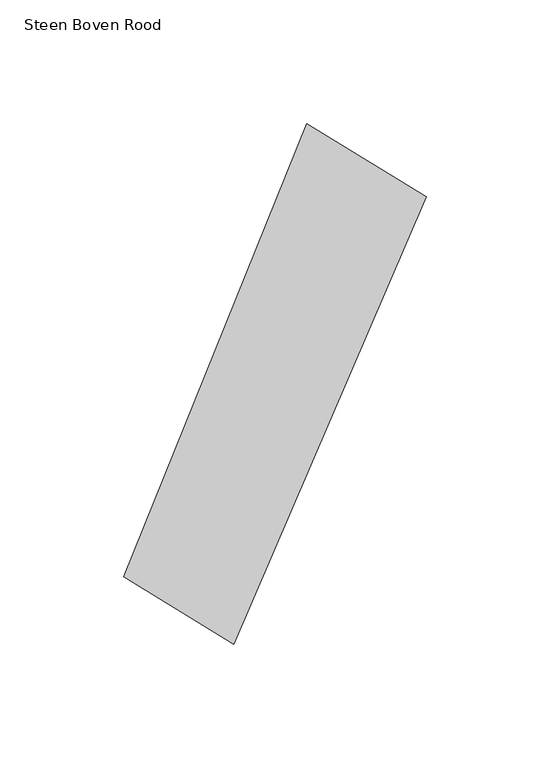
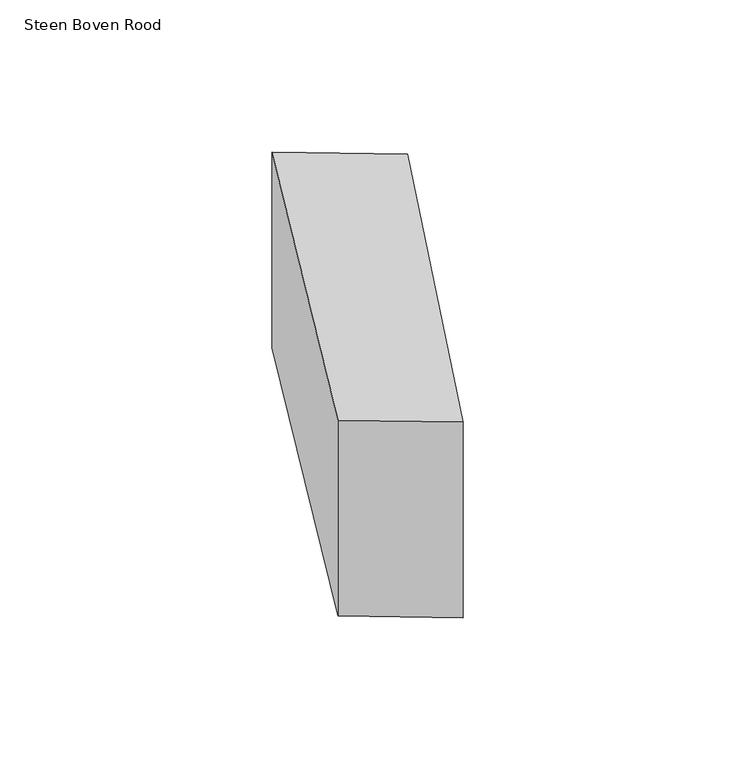
"""IFC4 building model written with IfcOpenShell, lengths in millimetres: proxy geometry, 00_GMA_steen_versie_4 : Steen Boven Rood."""

from ifc_helpers import new_model, si_unit, origin, origin_with_axes, place, context, project, spatial, polyline, outline, extrude, source, transform, mapped, element, save


def steen_boven_rood_8899d5ae(model_context):
    return source(origin(), model_context, "Body", "SweptSolid", [
        extrude(outline(polyline([(141.130172, 164.0549833), (63.4155416, -17.0520828), (18.763258, 10.2342014), (92.7848511, 193.615786), (141.130172, 164.0549833)])), origin_with_axes(), (0.0, 0.0, 1.0), 100.0),
    ])


if __name__ == "__main__":
    model = new_model("IFC4")
    model_context = context("Model", 3, world=origin())
    ifc_project = project(units=[si_unit("LENGTHUNIT", "METRE", prefix="MILLI")], contexts=[model_context])
    site = spatial("IfcSite", under=ifc_project)
    building = spatial("IfcBuilding", under=site)
    placement = place(None, origin())
    steen_boven_rood_shape = steen_boven_rood_8899d5ae(model_context)
    element("IfcBuildingElementProxy", 1, Name="00_GMA_steen_versie_4 : Steen Boven Rood", ObjectType="00_GMA_steen_versie_4 : Steen Boven Rood", at=placement, inside=building, context=model_context, shape_type="MappedRepresentation", body=[
        mapped(steen_boven_rood_shape, transform((0.0, 0.0, 0.0), x_axis=(1.0, 0.0, 0.0), y_axis=(0.0, 1.0, 0.0), z_axis=(0.0, 0.0, 1.0))),
    ])
    save(model, "model.ifc")

# Revit data of these elements
# Type "00_GMA_steen_versie_4 : Steen Boven Rood"
#   StootVoegHalfBoven [instance default] = 5 mm
#   StootVoegHalf [instance default] = 5 mm
#   StootVoegBreedteOnder = 10 mm
#   StootVoegBreedteBoven = 10 mm
#   Steendikte = 100 mm
#   LintVoegOnderHalf = 5 mm
#   LintVoegOnder = 10 mm
#   LintVoegBovenHalf = 0 mm
#   LintVoegBoven = 0 mm
#   materiaal = 21_steen_rood
#   MateriaalVoeg = none
#   Default Elevation = 0
# Element 1 (IfcBuildingElementProxy, "00_GMA_steen_versie_4 : Steen Boven Rood")
#   Materials on its faces: "21_steen_rood"
# Materials
#   "21_steen_rood": class "Unassigned", colour RGB 213 111 43, transparency 0, Cost = 0
